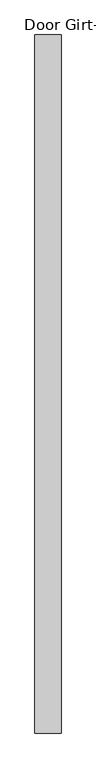
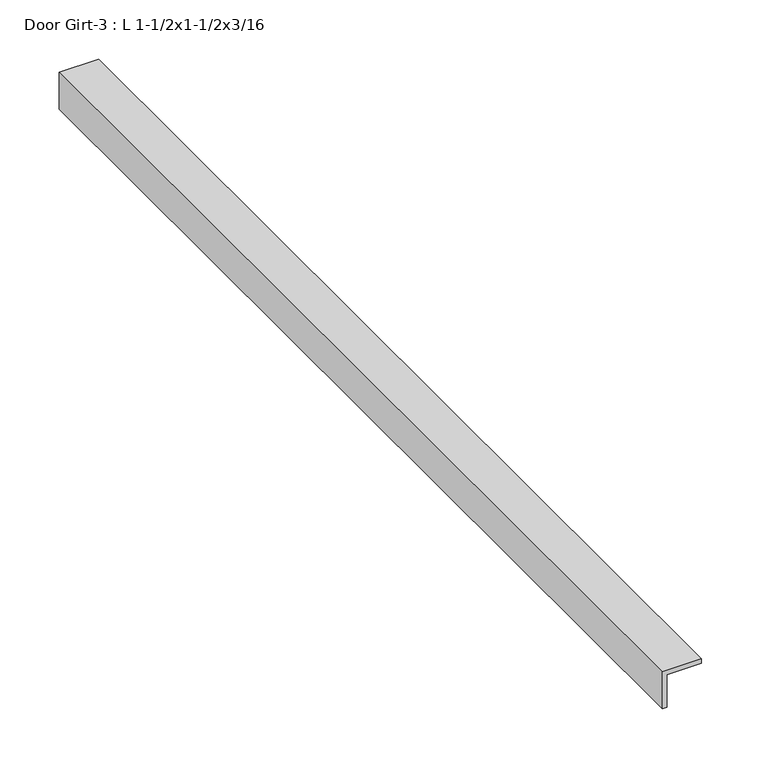
"""IFC4 building model written with IfcOpenShell, lengths in millimetres: proxy geometry, Door Girt-3 : L 1-1/2x1-1/2x3/16."""

from ifc_helpers import new_model, si_unit, frame, origin, place, context, project, spatial, polyline, outline, extrude, source, transform, mapped, element, save


def door_girt_3_l_1_1_2x1_1_2x3_16_18399394(model_context):
    return source(origin(), model_context, "Body", "SweptSolid", [
        extrude(outline(polyline([(812.8, 587403.9934739), (812.8, 587365.8934739), (774.7, 587365.8934739), (774.7, 587370.6559739), (808.0375, 587370.6559739), (808.0375, 587403.9934739), (812.8, 587403.9934739)])), frame((0.0, -533937.9163841, 0.0), z_axis=(0.0, 1.0, 0.0), x_axis=(0.0, 0.0, 1.0)), (0.0, 0.0, 1.0), 1016.0),
    ])


if __name__ == "__main__":
    model = new_model("IFC4")
    model_context = context("Model", 3, world=origin())
    ifc_project = project(units=[si_unit("LENGTHUNIT", "METRE", prefix="MILLI")], contexts=[model_context])
    site = spatial("IfcSite", under=ifc_project)
    building = spatial("IfcBuilding", under=site)
    placement = place(None, origin())
    door_girt_3_l_1_1_2x1_1_2x3_16_shape = door_girt_3_l_1_1_2x1_1_2x3_16_18399394(model_context)
    element("IfcBuildingElementProxy", 1, Name="Door Girt-3 : L 1-1/2x1-1/2x3/16", ObjectType="Door Girt-3 : L 1-1/2x1-1/2x3/16", at=placement, inside=building, context=model_context, shape_type="MappedRepresentation", body=[
        mapped(door_girt_3_l_1_1_2x1_1_2x3_16_shape, transform((0.0, 0.0, 0.0), x_axis=(1.0, 0.0, 0.0), y_axis=(0.0, 1.0, 0.0), z_axis=(0.0, 0.0, 1.0))),
    ])
    save(model, "model.ifc")

# Revit data of these elements
# Element 1 (IfcBuildingElementProxy, "Door Girt-3 : L 1-1/2x1-1/2x3/16")
#   Materials on its faces: "1-1/2\"X1-1/2\" GALV. STL L"
# Materials
#   "1-1/2\"X1-1/2\" GALV. STL L": class "Generic", colour RGB 211 211 207, transparency 0, Cost = 0
